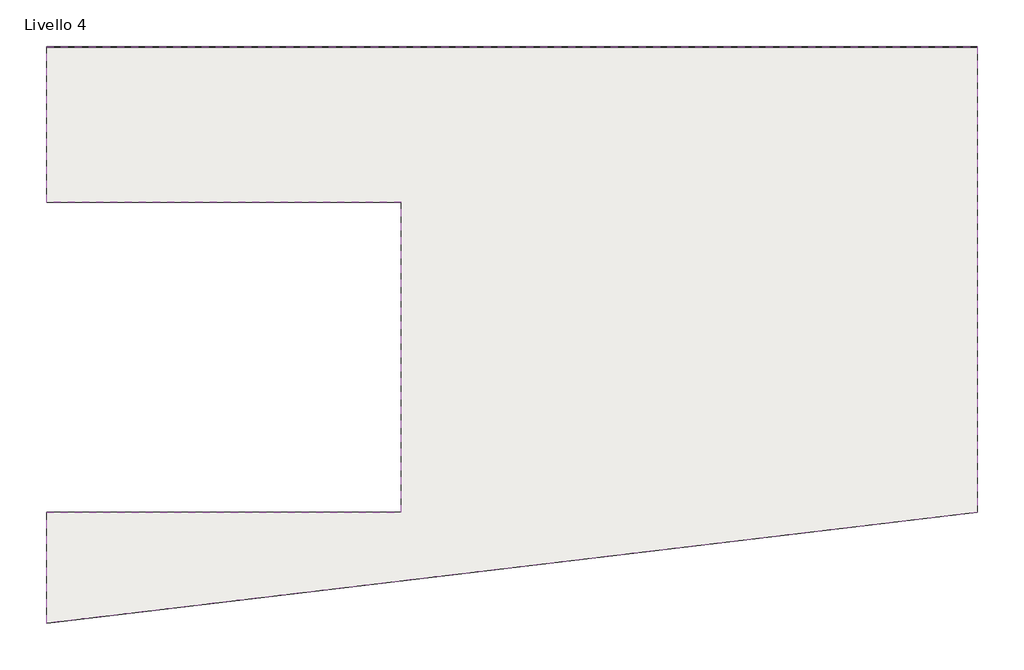
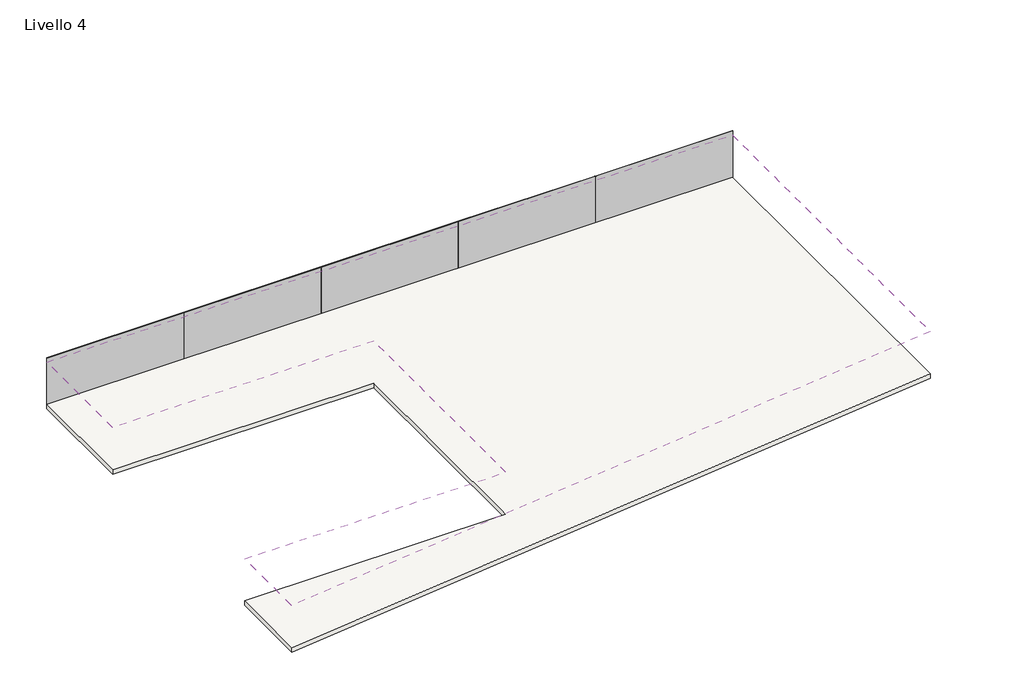
# One storey: 5 plates, 1 roof, 1 slab.
"""IFC4 building model written with IfcOpenShell, lengths in millimetres."""

import ifcopenshell
import ifcopenshell.guid

model = None  # the IFC model being written
_history = None  # IfcOwnerHistory: only IFC2X3 demands one
_inside = {}  # id of a spatial element -> (the spatial element, [elements in it])
_under = {}  # id of a project, library or spatial element -> (it, [spatial elements below it])
_declared = {}  # id of a project -> (the project, [libraries it declares])
_typed = {}  # id of a type object -> (the type object, [elements of that type])
_made_of = {}  # id of a material, layer set ... -> (it, [elements and type objects made of it])


def new_model(schema):
    """Start an empty IFC model of exactly this schema.

    Asked for "IFC4X3", IfcOpenShell would pick the latest addendum, in which some entities
    have other attributes; the version numbers below select the first issue.
    IFC2X3 requires an IfcOwnerHistory on every rooted entity: one is made here for all.
    """
    global model, _history
    if schema == "IFC4X3":
        model = ifcopenshell.file(schema_version=(4, 3, 0, 0))
    else:
        model = ifcopenshell.file(schema=schema)
    _inside.clear()
    _under.clear()
    _declared.clear()
    _typed.clear()
    _made_of.clear()
    _history = None
    if model.schema == "IFC2X3":
        org = make("IfcOrganization", Name="unknown")
        user = make(
            "IfcPersonAndOrganization",
            ThePerson=make("IfcPerson", FamilyName="unknown"),
            TheOrganization=org,
        )
        app = make(
            "IfcApplication",
            ApplicationDeveloper=org,
            Version="unknown",
            ApplicationFullName="unknown",
            ApplicationIdentifier="unknown",
        )
        _history = make(
            "IfcOwnerHistory",
            OwningUser=user,
            OwningApplication=app,
            ChangeAction="ADDED",
            CreationDate=0,
        )
    return model


def make(cls, **values):
    """One entity of the class cls with the attributes given. An attribute that is None is left unset."""
    return model.create_entity(
        cls, **{name: value for name, value in values.items() if value is not None}
    )


def rooted(cls, **values):
    """An entity with a GlobalId (a new one), such as an element, a storey or a relation."""
    return make(cls, GlobalId=ifcopenshell.guid.new(), OwnerHistory=_history, **values)


def si_unit(unit_type, name, prefix=None):
    """IfcSIUnit, for example si_unit("LENGTHUNIT", "METRE", prefix="MILLI")."""
    return make("IfcSIUnit", UnitType=unit_type, Prefix=prefix, Name=name)


def assignment(units):
    """IfcUnitAssignment: the units of a project."""
    return None if units is None else make("IfcUnitAssignment", Units=units)


def point(xyz):
    """IfcCartesianPoint."""
    return None if xyz is None else make("IfcCartesianPoint", Coordinates=xyz)


def direction(xyz):
    """IfcDirection."""
    return None if xyz is None else make("IfcDirection", DirectionRatios=xyz)


def frame(location, z_axis=None, x_axis=None):
    """IfcAxis2Placement3D, a coordinate frame: its origin and axes. An axis left out is left unset."""
    return make(
        "IfcAxis2Placement3D",
        Location=point(location),
        Axis=direction(z_axis),
        RefDirection=direction(x_axis),
    )


def origin():
    """The frame at (0, 0, 0) with its axes left unset."""
    return frame((0.0, 0.0, 0.0))


def origin_with_axes():
    """The frame at (0, 0, 0) with the z axis (0, 0, 1) and the x axis (1, 0, 0) written out."""
    return frame((0.0, 0.0, 0.0), z_axis=(0.0, 0.0, 1.0), x_axis=(1.0, 0.0, 0.0))


def place(relative_to, where):
    """IfcLocalPlacement: puts the frame where relative to a parent placement (None: the world)."""
    return make(
        "IfcLocalPlacement", PlacementRelTo=relative_to, RelativePlacement=where
    )


def context(
    kind, dimensions, precision=None, world=None, true_north=None, identifier=None
):
    """IfcGeometricRepresentationContext, for example the 3D "Model" context."""
    return make(
        "IfcGeometricRepresentationContext",
        ContextIdentifier=identifier,
        ContextType=kind,
        CoordinateSpaceDimension=dimensions,
        Precision=precision,
        WorldCoordinateSystem=world,
        TrueNorth=true_north,
    )


def project(units=None, contexts=None):
    """IfcProject with its units and contexts."""
    return rooted(
        "IfcProject",
        Name="project",
        RepresentationContexts=contexts,
        UnitsInContext=assignment(units),
    )


def spatial(cls, under=None, at=None, **own):
    """A site, building, storey or space (cls), placed at a placement, below another one or the project."""
    s = rooted(cls, ObjectPlacement=at, **own)
    if under is not None:
        _under.setdefault(under.id(), (under, []))[1].append(s)
    return s


def polyline(points):
    """IfcPolyline through the points."""
    return make("IfcPolyline", Points=[point(p) for p in points])


def outline(outer, holes=None, kind="AREA"):
    """IfcArbitraryClosedProfileDef: a profile drawn as a closed curve; with holes, ...WithVoids."""
    if holes is None:
        return make("IfcArbitraryClosedProfileDef", ProfileType=kind, OuterCurve=outer)
    return make(
        "IfcArbitraryProfileDefWithVoids",
        ProfileType=kind,
        OuterCurve=outer,
        InnerCurves=holes,
    )


def extrude(swept, where, along, depth):
    """IfcExtrudedAreaSolid: the profile swept, set in the frame where, extruded along a direction by depth."""
    return make(
        "IfcExtrudedAreaSolid",
        SweptArea=swept,
        Position=where,
        ExtrudedDirection=direction(along),
        Depth=depth,
    )


def faces_of(points, faces, orient=None, outer=None):
    """IfcFace entities. A face is a list of loops; a loop is a list of indices into points, from 0.

    orient and outer hold one flag for each loop. By default every Orientation is true, the
    first loop of a face is its IfcFaceOuterBound and the others are IfcFaceBound.
    """
    made = []
    for i, loops in enumerate(faces):
        bounds = []
        for j, loop in enumerate(loops):
            is_outer = j == 0 if outer is None else outer[i][j]
            bounds.append(
                make(
                    "IfcFaceOuterBound" if is_outer else "IfcFaceBound",
                    Bound=make("IfcPolyLoop", Polygon=[points[k] for k in loop]),
                    Orientation=True if orient is None else orient[i][j],
                )
            )
        made.append(make("IfcFace", Bounds=bounds))
    return made


def faceted_brep(points, faces, orient=None, outer=None, voids=None):
    """IfcFacetedBrep: a solid bounded by flat faces; with voids (closed shells), ...WithVoids."""
    shared = [point(p) for p in points]
    hull = make("IfcClosedShell", CfsFaces=faces_of(shared, faces, orient, outer))
    if voids is None:
        return make("IfcFacetedBrep", Outer=hull)
    return make(
        "IfcFacetedBrepWithVoids",
        Outer=hull,
        Voids=[
            make(cls, CfsFaces=faces_of(shared, fs, o, b)) for cls, fs, o, b in voids
        ],
    )


def shape(context_of_items, identifier, shape_type, items):
    """IfcShapeRepresentation: the items that make up one representation, for example the "Body"."""
    return make(
        "IfcShapeRepresentation",
        ContextOfItems=context_of_items,
        RepresentationIdentifier=identifier,
        RepresentationType=shape_type,
        Items=items,
    )


def source(mapping_origin, context_of_items, identifier, shape_type, items):
    """IfcRepresentationMap: a shape defined once, which mapped items show again and again."""
    return make(
        "IfcRepresentationMap",
        MappingOrigin=mapping_origin,
        MappedRepresentation=shape(context_of_items, identifier, shape_type, items),
    )


def transform(
    local_origin,
    x_axis=None,
    y_axis=None,
    z_axis=None,
    scale=None,
    scale2=None,
    scale3=None,
    uniform=True,
):
    """IfcCartesianTransformationOperator3D, or its non-uniform kind. x_axis, y_axis, z_axis: its Axis1, 2, 3."""
    if uniform:
        return make(
            "IfcCartesianTransformationOperator3D",
            Axis1=direction(x_axis),
            Axis2=direction(y_axis),
            LocalOrigin=point(local_origin),
            Scale=scale,
            Axis3=direction(z_axis),
        )
    return make(
        "IfcCartesianTransformationOperator3DnonUniform",
        Axis1=direction(x_axis),
        Axis2=direction(y_axis),
        LocalOrigin=point(local_origin),
        Scale=scale,
        Axis3=direction(z_axis),
        Scale2=scale2,
        Scale3=scale3,
    )


def mapped(mapping_source, mapping_target):
    """IfcMappedItem: shows the shape of a source again, moved by a transform."""
    return make(
        "IfcMappedItem", MappingSource=mapping_source, MappingTarget=mapping_target
    )


def made_of(thing, what):
    """Note that an element or type object is made of a material, layer set ...; save() writes the relation."""
    if what is not None:
        _made_of.setdefault(what.id(), (what, []))[1].append(thing)
    return thing


def element(
    cls,
    number,
    at=None,
    inside=None,
    cuts=None,
    type_object=None,
    material=None,
    context=None,
    identifier="Body",
    shape_type=None,
    held_by="IfcProductDefinitionShape",
    body=None,
    shapes=None,
    **own,
):
    """One element of the class cls, such as IfcWall. Its Tag is "e" and its number.

    at: its placement. inside: the storey or other place that contains it. cuts: it is an
    opening in that element (IfcRelVoidsElement). A single representation is given by context,
    identifier, shape_type and body (its items); several are given by shapes. held_by: the class
    of the entity that holds the representations. save() writes the other relations.
    """
    e = rooted(cls, Tag="e%d" % number, ObjectPlacement=at, **own)
    if body is not None:
        shapes = [shape(context, identifier, shape_type, body)]
    if shapes is not None:
        e.Representation = make(held_by, Representations=shapes)
    if inside is not None:
        _inside.setdefault(inside.id(), (inside, []))[1].append(e)
    if cuts is not None:
        rooted(
            "IfcRelVoidsElement", RelatingBuildingElement=cuts, RelatedOpeningElement=e
        )
    if type_object is not None:
        _typed.setdefault(type_object.id(), (type_object, []))[1].append(e)
    return made_of(e, material)


def aggregate(whole, parts):
    """IfcRelAggregates: a whole, such as a stair, and the parts it consists of."""
    return rooted("IfcRelAggregates", RelatingObject=whole, RelatedObjects=parts)


def save(model, path):
    """Write the relations noted so far, then the file.

    IfcRelAggregates (storeys below a building ...), IfcRelContainedInSpatialStructure (elements
    in a storey), IfcRelDefinesByType, IfcRelAssociatesMaterial and IfcRelDeclares: one each for
    every whole, place, type object, material and project.
    """
    for whole, parts in _under.values():
        aggregate(whole, parts)
    for where, things in _inside.values():
        rooted(
            "IfcRelContainedInSpatialStructure",
            RelatedElements=things,
            RelatingStructure=where,
        )
    for kind, things in _typed.values():
        rooted("IfcRelDefinesByType", RelatedObjects=things, RelatingType=kind)
    for what, things in _made_of.values():
        rooted("IfcRelAssociatesMaterial", RelatedObjects=things, RelatingMaterial=what)
    for by, libraries in _declared.values():
        rooted("IfcRelDeclares", RelatingContext=by, RelatedDefinitions=libraries)
    model.write(path)


def pannello_sistema_vetrato_29ff3466(model_context):
    return source(origin(), model_context, "Body", "SweptSolid", [
        extrude(outline(polyline([(4200.0000001, -15.0), (-4200.0000001, -15.0), (-4200.0000001, 15.0), (4200.0000001, 15.0), (4200.0000001, -15.0)])), origin_with_axes(), (0.0, 0.0, 1.0), 3000.0),
    ])


model = new_model("IFC4")

# Units and contexts
model_context = context("Model", 3, world=origin())
ifc_project = project(units=[si_unit("LENGTHUNIT", "METRE", prefix="MILLI")], contexts=[model_context])

# Site, building, storey
site = spatial("IfcSite", under=ifc_project)
building = spatial("IfcBuilding", under=site)
storey = spatial("IfcBuildingStorey", under=building, Name="Livello 4", Elevation=12000.0)

# Plates
placement = place(None, origin())
pannello_sistema_vetrato_shape = pannello_sistema_vetrato_29ff3466(model_context)
element("IfcPlate", 1, ObjectType="Pannello sistema : Vetrato", at=placement, inside=storey, context=model_context, shape_type="MappedRepresentation", body=[
    mapped(pannello_sistema_vetrato_shape, transform((-20934.9893485, 13197.4454735, 12000.0), x_axis=(1.0, 0.0, 0.0), y_axis=(0.0, 1.0, 0.0), z_axis=(0.0, 0.0, 1.0))),
])
element("IfcPlate", 2, ObjectType="Pannello sistema : Vetrato", at=placement, inside=storey, context=model_context, shape_type="MappedRepresentation", body=[
    mapped(pannello_sistema_vetrato_shape, transform((-12534.9893485, 13197.4454735, 12000.0), x_axis=(1.0, 0.0, 0.0), y_axis=(0.0, 1.0, 0.0), z_axis=(0.0, 0.0, 1.0))),
])
element("IfcPlate", 3, ObjectType="Pannello sistema : Vetrato", at=placement, inside=storey, context=model_context, shape_type="MappedRepresentation", body=[
    mapped(pannello_sistema_vetrato_shape, transform((-4134.9893486, 13197.4454735, 12000.0), x_axis=(1.0, 0.0, 0.0), y_axis=(0.0, 1.0, 0.0), z_axis=(0.0, 0.0, 1.0))),
])
element("IfcPlate", 4, ObjectType="Pannello sistema : Vetrato", at=placement, inside=storey, context=model_context, shape_type="MappedRepresentation", body=[
    mapped(pannello_sistema_vetrato_shape, transform((4265.0106513, 13197.4454735, 12000.0), x_axis=(1.0, 0.0, 0.0), y_axis=(0.0, 1.0, 0.0), z_axis=(0.0, 0.0, 1.0))),
])
element("IfcPlate", 5, ObjectType="Pannello sistema : Vetrato", at=placement, inside=storey, context=model_context, shape_type="MappedRepresentation", body=[
    mapped(pannello_sistema_vetrato_shape, transform((12665.0106513, 13197.4454735, 12000.0), x_axis=(1.0, 0.0, 0.0), y_axis=(0.0, 1.0, 0.0), z_axis=(0.0, 0.0, 1.0))),
])

# Roof
element("IfcRoof", 6, ObjectType="Latero Cementizio - 27 cm", at=placement, inside=storey, context=model_context, shape_type="Brep", body=[
    faceted_brep([(16865.0106514, -7802.5545265, 14730.0), (16865.0106514, -7802.5545265, 15000.0), (-25134.9893486, -12802.5545265, 15000.0), (-25134.9893486, -12802.5545265, 14730.0), (-25134.9893486, -7802.5545265, 15000.0), (-25134.9893486, -7802.5545265, 14730.0), (-9134.9893486, -7802.5545265, 20455.4928107), (-9134.9893486, -7802.5545265, 20185.4928107), (-9134.9893486, 6197.4454735, 20028.9385911), (-9134.9893486, 6197.4454735, 19758.9385911), (-25134.9893486, 6197.4454735, 15000.0), (-25134.9893486, 6197.4454735, 14730.0), (-25134.9893486, 13197.4454735, 15000.0), (-25134.9893486, 13197.4454735, 14730.0), (16865.0106514, 13197.4454735, 15000.0), (16865.0106514, 13197.4454735, 14730.0)], [[[0, 1, 2, 3]], [[3, 2, 4, 5]], [[5, 4, 6, 7]], [[7, 6, 8, 9]], [[9, 8, 10, 11]], [[11, 10, 12, 13]], [[13, 12, 14, 15]], [[15, 14, 1, 0]], [[1, 14, 8]], [[0, 9, 15]], [[6, 4, 2]], [[1, 8, 6]], [[1, 6, 2]], [[7, 3, 5]], [[0, 7, 9]], [[0, 3, 7]], [[12, 10, 8]], [[14, 12, 8]], [[13, 9, 11]], [[15, 9, 13]]]),
])

# Slab
element("IfcSlab", 7, ObjectType="Latero Cementizio - 30 cm", at=placement, inside=storey, context=model_context, shape_type="SweptSolid", body=[
    extrude(outline(polyline([(-25134.9893486, -7802.5545265), (-9134.9893486, -7802.5545265), (-9134.9893486, 6197.4454735), (-25134.9893486, 6197.4454735), (-25134.9893486, 13197.4454735), (16865.0106514, 13197.4454735), (16865.0106514, -7802.5545265), (-25134.9893486, -12802.5545265), (-25134.9893486, -7802.5545265)])), frame((0.0, 0.0, 11700.0), z_axis=(0.0, 0.0, 1.0), x_axis=(1.0, 0.0, 0.0)), (0.0, 0.0, 1.0), 300.0),
])

save(model, "model.ifc")

# Revit data of these elements
# Type "Pannello sistema : Vetrato"
#   Construction Type Id = "GSP4R"
#   Analytic Construction = "Vetrata singola Pilkington 1/8 in"
#   Visual Light Transmittance = 0.9
#   Solar Heat Gain Coefficient = 0.86
#   Heat Transfer Coefficient (U) = 6.7069 W/(m²·K)
# Type "Latero Cementizio - 27 cm"
#   Keynote = "T/1"
#   Layers, outside or top first: 0.05 m "Coppi" (function 4); 0.04 m "Calcestruzzo" (function 2); 0.16 m "Laterizio (2)" (function 1); 0.02 m "Intonaco - Bianco" (function 5)
# Type "Latero Cementizio - 30 cm"
#   Keynote = "S/3"
#   Function = 0
#   Layers, outside or top first: 0.02 m "Ceramica bianca" (function 4); 0.065 m "Sabbia e Calcestruzzo" (function 2); 0.04 m "Calcestruzzo" (function 1); 0.16 m "Laterizio (2)" (function 1); 0.015 m "Intonaco - Bianco" (function 5)
# Elements 1, 2, 3, 4, 5 (IfcPlate, "Pannello sistema : Vetrato")
#   Phase Created = Stato di Progetto
#   Materials on its faces: "Default - Vetro"
# Element 6 (IfcRoof, "Latero Cementizio - 27 cm")
#   built-in parameter 1001710 = 33615
#   Phase Created = Stato di Progetto
#   Materials on its faces: "Intonaco - Bianco", "Coppi"
# Element 7 (IfcSlab, "Latero Cementizio - 30 cm")
#   built-in parameter 1001955 = 1.5708 (stored number, unit not read)
#   Height Offset From Level = 0.00 m
#   Phase Created = Stato di Progetto
#   Materials on its faces: "Intonaco - Bianco", "Ceramica bianca"
# Materials
#   "Coppi": class "Varie", colour RGB 194 100 86, transparency 0, Description = "Tegole in mattone", Cost = 0
#   "Calcestruzzo": class "Calcestruzzo", colour RGB 192 192 192, transparency 0, Description = "Calcestruzzo - Cemento Portland", Cost = 0
#   "Laterizio (2)": class "Mattone", colour RGB 255 128 64, transparency 0, Description = "Pignatta h 16 cm", Cost = 0
#   "Intonaco - Bianco": class "Intonaco", colour RGB 249 249 249, transparency 0, Description = "Verniciatura", Cost = 0
#   "Ceramica bianca": class "Ceramica", colour RGB 210 210 210, transparency 0, Description = "Finitura interna - Piastrelle di ceramica incollate", Cost = 0
#   "Sabbia e Calcestruzzo": class "Calcestruzzo", colour RGB 127 127 127, transparency 0, Description = "Magrone - Sabbia e cemento", Cost = 0
#   "Default - Vetro": class "Vetro", colour RGB 208 208 208, transparency 0.7, Cost = 0
